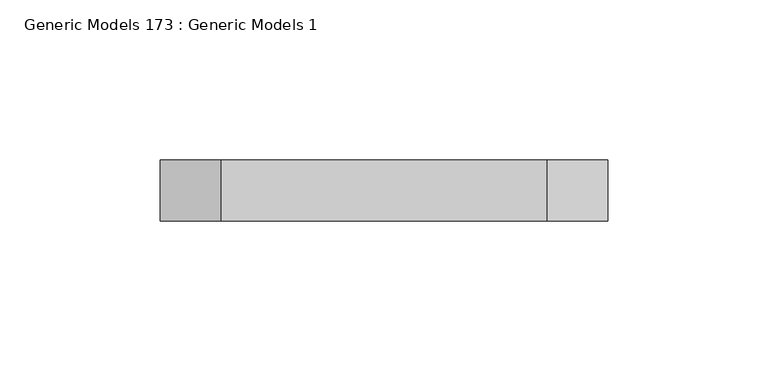
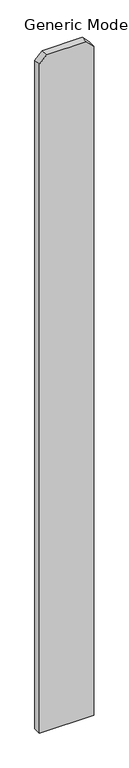
"""IFC4 building model written with IfcOpenShell, lengths in millimetres: proxy geometry, Generic Models 173 : Generic Models 1."""

from ifc_helpers import new_model, si_unit, frame, origin, place, context, project, spatial, polyline, outline, extrude, source, transform, mapped, element, save


def generic_models_173_generic_models_1_7547f4db(model_context):
    return source(origin(), model_context, "Body", "SweptSolid", [
        extrude(outline(polyline([(76.2, 56361.0125), (1885.95, 56361.0125), (1905.0, 56341.9625), (1905.0, 56240.3625), (1885.95, 56221.3125), (76.2, 56221.3125), (76.2, 56361.0125)])), frame((0.0, 547.6875, 0.0), z_axis=(0.0, 1.0, 0.0), x_axis=(0.0, 0.0, 1.0)), (0.0, 0.0, 1.0), 19.05),
    ])


if __name__ == "__main__":
    model = new_model("IFC4")
    model_context = context("Model", 3, world=origin())
    ifc_project = project(units=[si_unit("LENGTHUNIT", "METRE", prefix="MILLI")], contexts=[model_context])
    site = spatial("IfcSite", under=ifc_project)
    building = spatial("IfcBuilding", under=site)
    placement = place(None, origin())
    generic_models_173_generic_models_1_shape = generic_models_173_generic_models_1_7547f4db(model_context)
    element("IfcBuildingElementProxy", 1, Name="Generic Models 173 : Generic Models 1", ObjectType="Generic Models 173 : Generic Models 1", at=placement, inside=building, context=model_context, shape_type="MappedRepresentation", body=[
        mapped(generic_models_173_generic_models_1_shape, transform((0.0, 0.0, 0.0), x_axis=(1.0, 0.0, 0.0), y_axis=(0.0, 1.0, 0.0), z_axis=(0.0, 0.0, 1.0))),
    ])
    save(model, "model.ifc")

# Revit data of these elements
# Element 1 (IfcBuildingElementProxy, "Generic Models 173 : Generic Models 1")
#   Materials on its faces: "VERTICAL 1X6 CEDAR PLANKS W/ CLEAR WOOD SEALER"
# Materials
#   "VERTICAL 1X6 CEDAR PLANKS W/ CLEAR WOOD SEALER": class "Wood", colour RGB 234 198 147, transparency 0, Description = "Pinus Echinata", Cost = 0
